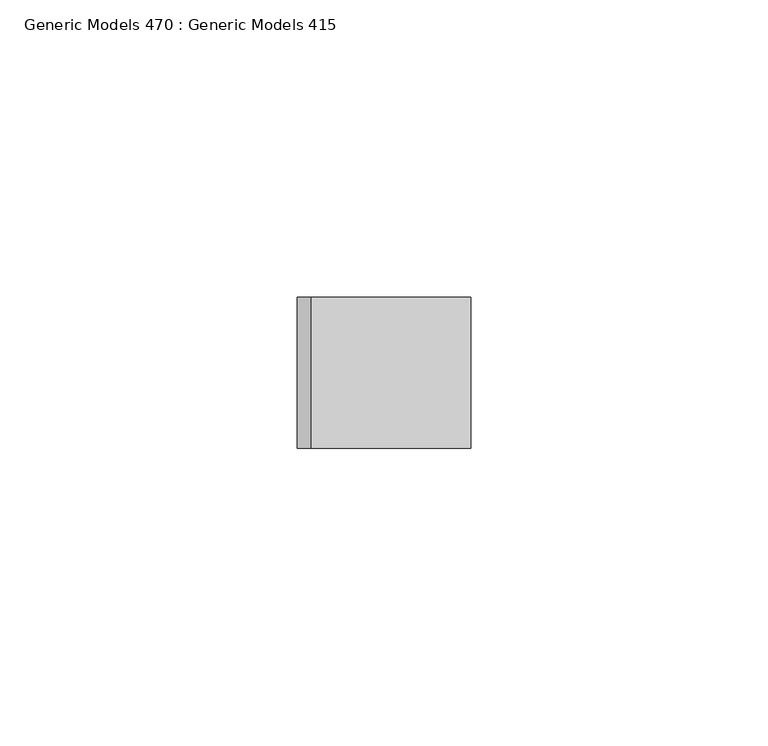
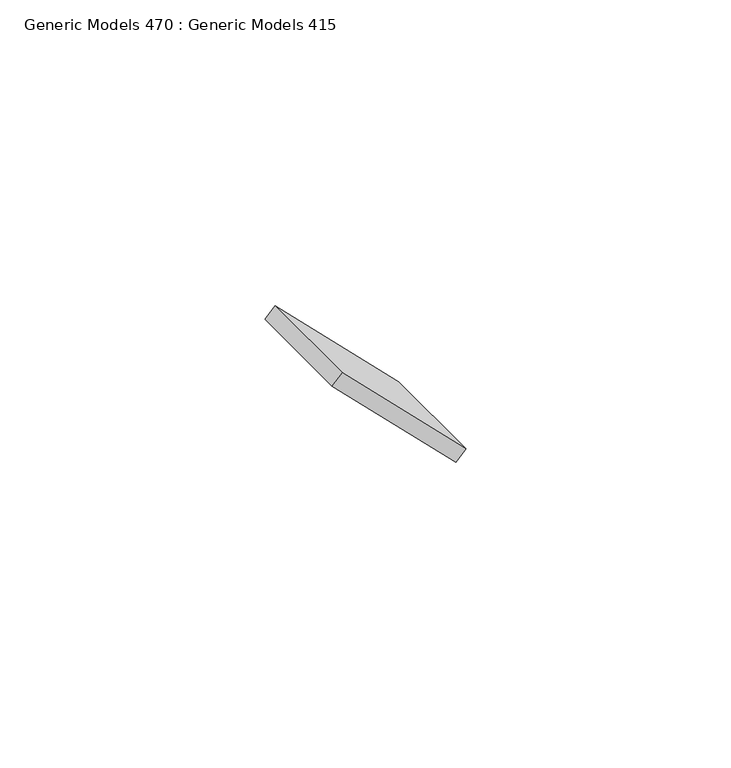
"""IFC4 building model written with IfcOpenShell, lengths in millimetres: proxy geometry, Generic Models 470 : Generic Models 415."""

from ifc_helpers import new_model, si_unit, frame, origin, place, context, project, spatial, polyline, outline, extrude, source, transform, mapped, element, save


def generic_models_470_generic_models_415_ec80f388(model_context):
    return source(origin(), model_context, "Body", "SweptSolid", [
        extrude(outline(polyline([(0.0, -38.1), (0.0, 0.0), (25.4, 0.0), (25.4, -38.1), (0.0, -38.1)])), frame((-6869.8996186, -4475.9863946, 128162.5002957), z_axis=(0.7071067811864907, 0.0, 0.7071067811866044), x_axis=(0.0, -1.0, 0.0)), (0.0, 0.0, 1.0), 3.175),
    ])


if __name__ == "__main__":
    model = new_model("IFC4")
    model_context = context("Model", 3, world=origin())
    ifc_project = project(units=[si_unit("LENGTHUNIT", "METRE", prefix="MILLI")], contexts=[model_context])
    site = spatial("IfcSite", under=ifc_project)
    building = spatial("IfcBuilding", under=site)
    placement = place(None, origin())
    generic_models_470_generic_models_415_shape = generic_models_470_generic_models_415_ec80f388(model_context)
    element("IfcBuildingElementProxy", 1, Name="Generic Models 470 : Generic Models 415", ObjectType="Generic Models 470 : Generic Models 415", at=placement, inside=building, context=model_context, shape_type="MappedRepresentation", body=[
        mapped(generic_models_470_generic_models_415_shape, transform((0.0, 0.0, 0.0), x_axis=(1.0, 0.0, 0.0), y_axis=(0.0, 1.0, 0.0), z_axis=(0.0, 0.0, 1.0))),
    ])
    save(model, "model.ifc")

# Revit data of these elements
# Element 1 (IfcBuildingElementProxy, "Generic Models 470 : Generic Models 415")
#   Materials on its faces: "_WELDED STEEL TABS FOR LOUVER ATTACHMENT"
# Materials
#   "_WELDED STEEL TABS FOR LOUVER ATTACHMENT": class "Metal", colour RGB 199 199 199, transparency 0, Description = "Structural steel 50ksi", Cost = 0
